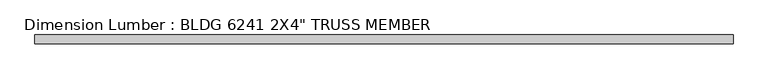
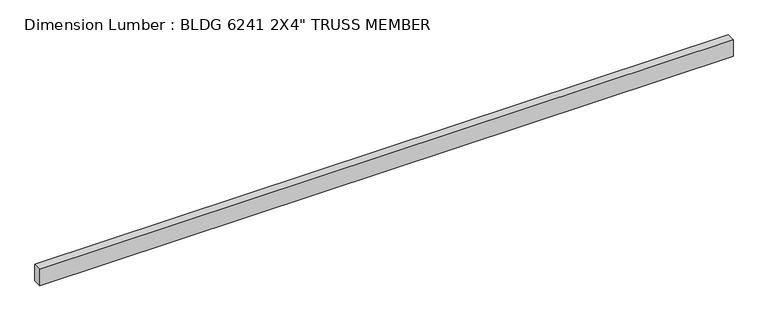
"""IFC4 building model written with IfcOpenShell, lengths in millimetres: beam geometry."""

from ifc_helpers import new_model, si_unit, frame, origin, place, context, project, spatial, polyline, outline, extrude, source, transform, mapped, element, save


def beam_d87feb12(model_context):
    return source(origin(), model_context, "Body", "SweptSolid", [
        extrude(outline(polyline([(2032.0, 25.4), (2032.0, -25.4), (-2032.0, -25.4), (-2032.0, 25.4), (2032.0, 25.4)])), frame((0.0, 0.0, -50.8), z_axis=(0.0, 0.0, 1.0), x_axis=(1.0, 0.0, 0.0)), (0.0, 0.0, 1.0), 101.6),
    ])


if __name__ == "__main__":
    model = new_model("IFC4")
    model_context = context("Model", 3, world=origin())
    ifc_project = project(units=[si_unit("LENGTHUNIT", "METRE", prefix="MILLI")], contexts=[model_context])
    site = spatial("IfcSite", under=ifc_project)
    building = spatial("IfcBuilding", under=site)
    placement = place(None, origin())
    beam_shape = beam_d87feb12(model_context)
    element("IfcBeam", 1, ObjectType="Dimension Lumber : BLDG 6241 2X4\" TRUSS MEMBER", at=placement, inside=building, context=model_context, shape_type="MappedRepresentation", body=[
        mapped(beam_shape, transform((0.0, 0.0, 0.0), x_axis=(1.0, 0.0, 0.0), y_axis=(0.0, 1.0, 0.0), z_axis=(0.0, 0.0, 1.0))),
    ])
    save(model, "model.ifc")

# Revit data of these elements
# Type "Dimension Lumber : BLDG 6241 2X4\" TRUSS MEMBER"
#   Assembly Code = "B10"
#   A = 0.273472 SF
#   Length [instance default] = 5' - 0"
#   b = 0' - 2"
#   d = 0' - 4"
#   Structural Material [instance default] = Softwood, Lumber
# Element 1 (IfcBeam, "Dimension Lumber : BLDG 6241 2X4\" TRUSS MEMBER")
#   Materials on its faces: "Softwood, Lumber"
# Materials
#   "Softwood, Lumber": class "Wood", colour RGB 223 192 134, transparency 0, Description = "Pinus Echinata", Cost = 0
